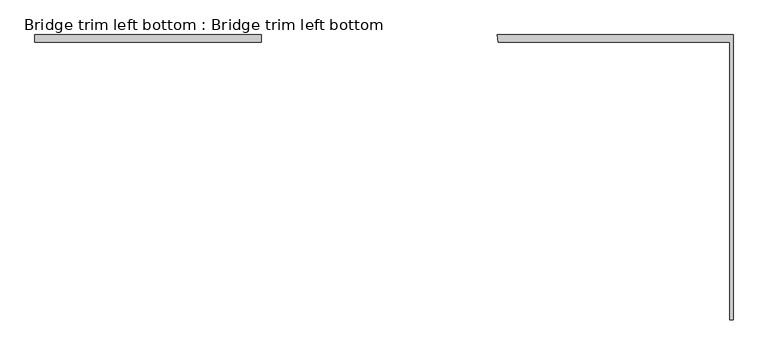
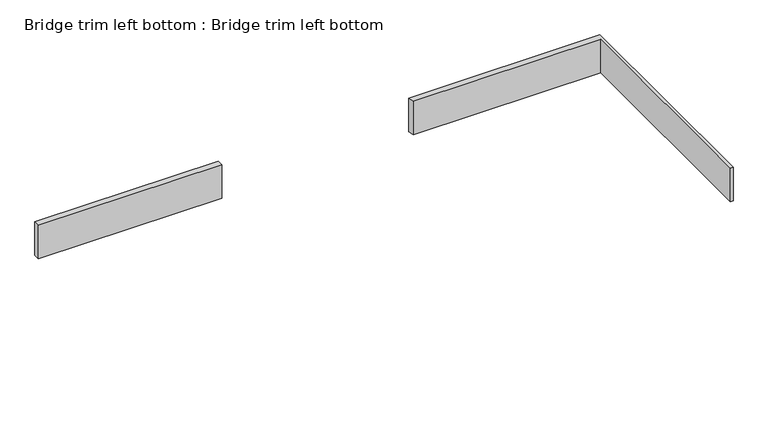
"""IFC4 building model written with IfcOpenShell, lengths in millimetres: furniture geometry, Bridge trim left bottom : Bridge trim left bottom."""

from ifc_helpers import new_model, si_unit, frame, origin, place, context, project, spatial, polyline, outline, extrude, source, transform, mapped, element, save


def bridge_trim_left_bottom_bridge_trim_left_bottom_b1ceb173(model_context):
    return source(origin(), model_context, "Body", "SweptSolid", [
        extrude(outline(polyline([(103.1875, 11912.6), (103.1875, 11857.0375), (-1578.305012, 11857.0375), (-1578.305012, 11912.6), (-1537.194945, 11912.6), (103.1875, 11912.6)])), frame((0.0, 0.0, 2717.8), z_axis=(0.0, 0.0, 1.0), x_axis=(1.0, 0.0, 0.0)), (0.0, 0.0, 1.0), 323.85),
        extrude(outline(polyline([(3606.0306594, 11912.6), (3606.0306594, 9793.2875), (3580.6306594, 9793.2875), (3580.6306594, 11857.0375), (1860.55, 11857.0375), (1853.4306594, 11912.6), (3606.0306594, 11912.6)])), frame((0.0, 0.0, 2717.8), z_axis=(0.0, 0.0, 1.0), x_axis=(1.0, 0.0, 0.0)), (0.0, 0.0, 1.0), 323.85),
    ])


if __name__ == "__main__":
    model = new_model("IFC4")
    model_context = context("Model", 3, world=origin())
    ifc_project = project(units=[si_unit("LENGTHUNIT", "METRE", prefix="MILLI")], contexts=[model_context])
    site = spatial("IfcSite", under=ifc_project)
    building = spatial("IfcBuilding", under=site)
    placement = place(None, origin())
    bridge_trim_left_bottom_bridge_trim_left_bottom_shape = bridge_trim_left_bottom_bridge_trim_left_bottom_b1ceb173(model_context)
    element("IfcFurniture", 1, ObjectType="Bridge trim left bottom : Bridge trim left bottom", at=placement, inside=building, context=model_context, shape_type="MappedRepresentation", body=[
        mapped(bridge_trim_left_bottom_bridge_trim_left_bottom_shape, transform((0.0, 0.0, 0.0), x_axis=(1.0, 0.0, 0.0), y_axis=(0.0, 1.0, 0.0), z_axis=(0.0, 0.0, 1.0))),
    ])
    save(model, "model.ifc")

# Revit data of these elements
# Type "Bridge trim left bottom : Bridge trim left bottom"
#   COBie.Type = no
# Element 1 (IfcFurniture, "Bridge trim left bottom : Bridge trim left bottom")
#   Materials on its faces: "Trim - White"
# Materials
#   "Trim - White": class "Wood", colour RGB 255 255 255, transparency 0, Cost = 0
